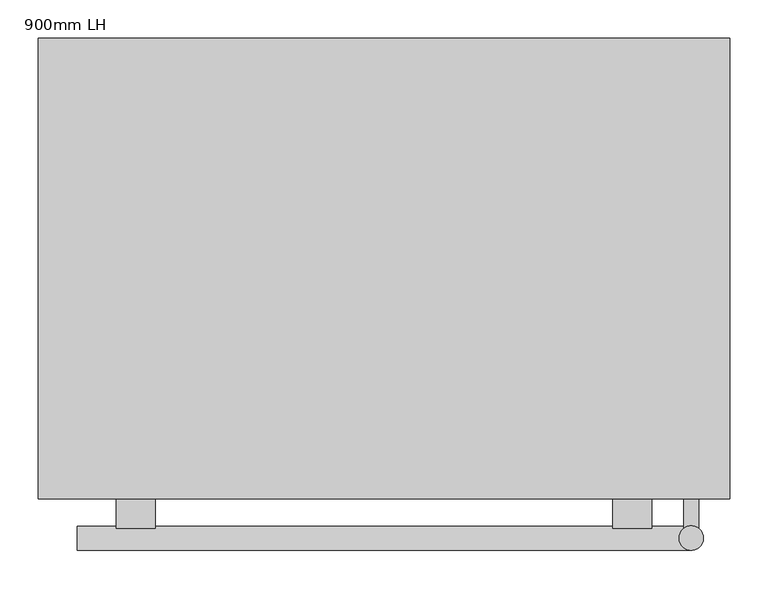
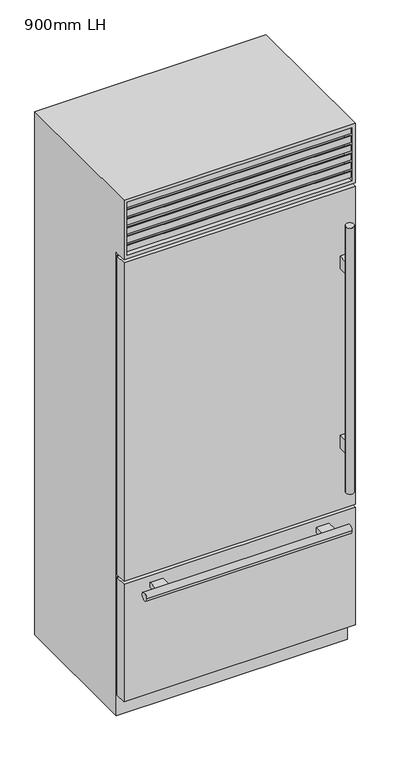
"""IFC4 building model written with IfcOpenShell, lengths in millimetres: proxy geometry, Refrigerador-combinado : 900mm LH."""

import ifcopenshell
import ifcopenshell.guid

model = None  # the IFC model being written
_history = None  # IfcOwnerHistory: only IFC2X3 demands one
_inside = {}  # id of a spatial element -> (the spatial element, [elements in it])
_under = {}  # id of a project, library or spatial element -> (it, [spatial elements below it])
_declared = {}  # id of a project -> (the project, [libraries it declares])
_typed = {}  # id of a type object -> (the type object, [elements of that type])
_made_of = {}  # id of a material, layer set ... -> (it, [elements and type objects made of it])


def new_model(schema):
    """Start an empty IFC model of exactly this schema.

    Asked for "IFC4X3", IfcOpenShell would pick the latest addendum, in which some entities
    have other attributes; the version numbers below select the first issue.
    IFC2X3 requires an IfcOwnerHistory on every rooted entity: one is made here for all.
    """
    global model, _history
    if schema == "IFC4X3":
        model = ifcopenshell.file(schema_version=(4, 3, 0, 0))
    else:
        model = ifcopenshell.file(schema=schema)
    _inside.clear()
    _under.clear()
    _declared.clear()
    _typed.clear()
    _made_of.clear()
    _history = None
    if model.schema == "IFC2X3":
        org = make("IfcOrganization", Name="unknown")
        user = make(
            "IfcPersonAndOrganization",
            ThePerson=make("IfcPerson", FamilyName="unknown"),
            TheOrganization=org,
        )
        app = make(
            "IfcApplication",
            ApplicationDeveloper=org,
            Version="unknown",
            ApplicationFullName="unknown",
            ApplicationIdentifier="unknown",
        )
        _history = make(
            "IfcOwnerHistory",
            OwningUser=user,
            OwningApplication=app,
            ChangeAction="ADDED",
            CreationDate=0,
        )
    return model


def make(cls, **values):
    """One entity of the class cls with the attributes given. An attribute that is None is left unset."""
    return model.create_entity(
        cls, **{name: value for name, value in values.items() if value is not None}
    )


def rooted(cls, **values):
    """An entity with a GlobalId (a new one), such as an element, a storey or a relation."""
    return make(cls, GlobalId=ifcopenshell.guid.new(), OwnerHistory=_history, **values)


def si_unit(unit_type, name, prefix=None):
    """IfcSIUnit, for example si_unit("LENGTHUNIT", "METRE", prefix="MILLI")."""
    return make("IfcSIUnit", UnitType=unit_type, Prefix=prefix, Name=name)


def assignment(units):
    """IfcUnitAssignment: the units of a project."""
    return None if units is None else make("IfcUnitAssignment", Units=units)


def point(xyz):
    """IfcCartesianPoint."""
    return None if xyz is None else make("IfcCartesianPoint", Coordinates=xyz)


def direction(xyz):
    """IfcDirection."""
    return None if xyz is None else make("IfcDirection", DirectionRatios=xyz)


def frame(location, z_axis=None, x_axis=None):
    """IfcAxis2Placement3D, a coordinate frame: its origin and axes. An axis left out is left unset."""
    return make(
        "IfcAxis2Placement3D",
        Location=point(location),
        Axis=direction(z_axis),
        RefDirection=direction(x_axis),
    )


def origin():
    """The frame at (0, 0, 0) with its axes left unset."""
    return frame((0.0, 0.0, 0.0))


def place(relative_to, where):
    """IfcLocalPlacement: puts the frame where relative to a parent placement (None: the world)."""
    return make(
        "IfcLocalPlacement", PlacementRelTo=relative_to, RelativePlacement=where
    )


def context(
    kind, dimensions, precision=None, world=None, true_north=None, identifier=None
):
    """IfcGeometricRepresentationContext, for example the 3D "Model" context."""
    return make(
        "IfcGeometricRepresentationContext",
        ContextIdentifier=identifier,
        ContextType=kind,
        CoordinateSpaceDimension=dimensions,
        Precision=precision,
        WorldCoordinateSystem=world,
        TrueNorth=true_north,
    )


def project(units=None, contexts=None):
    """IfcProject with its units and contexts."""
    return rooted(
        "IfcProject",
        Name="project",
        RepresentationContexts=contexts,
        UnitsInContext=assignment(units),
    )


def spatial(cls, under=None, at=None, **own):
    """A site, building, storey or space (cls), placed at a placement, below another one or the project."""
    s = rooted(cls, ObjectPlacement=at, **own)
    if under is not None:
        _under.setdefault(under.id(), (under, []))[1].append(s)
    return s


def polyline(points):
    """IfcPolyline through the points."""
    return make("IfcPolyline", Points=[point(p) for p in points])


def circle_curve(where, radius):
    """IfcCircle in the frame where."""
    return make("IfcCircle", Position=where, Radius=radius)


def ellipse_curve(where, semi_axis1, semi_axis2):
    """IfcEllipse in the frame where."""
    return make(
        "IfcEllipse", Position=where, SemiAxis1=semi_axis1, SemiAxis2=semi_axis2
    )


def outline(outer, holes=None, kind="AREA"):
    """IfcArbitraryClosedProfileDef: a profile drawn as a closed curve; with holes, ...WithVoids."""
    if holes is None:
        return make("IfcArbitraryClosedProfileDef", ProfileType=kind, OuterCurve=outer)
    return make(
        "IfcArbitraryProfileDefWithVoids",
        ProfileType=kind,
        OuterCurve=outer,
        InnerCurves=holes,
    )


def extrude(swept, where, along, depth):
    """IfcExtrudedAreaSolid: the profile swept, set in the frame where, extruded along a direction by depth."""
    return make(
        "IfcExtrudedAreaSolid",
        SweptArea=swept,
        Position=where,
        ExtrudedDirection=direction(along),
        Depth=depth,
    )


def faces_of(points, faces, orient=None, outer=None):
    """IfcFace entities. A face is a list of loops; a loop is a list of indices into points, from 0.

    orient and outer hold one flag for each loop. By default every Orientation is true, the
    first loop of a face is its IfcFaceOuterBound and the others are IfcFaceBound.
    """
    made = []
    for i, loops in enumerate(faces):
        bounds = []
        for j, loop in enumerate(loops):
            is_outer = j == 0 if outer is None else outer[i][j]
            bounds.append(
                make(
                    "IfcFaceOuterBound" if is_outer else "IfcFaceBound",
                    Bound=make("IfcPolyLoop", Polygon=[points[k] for k in loop]),
                    Orientation=True if orient is None else orient[i][j],
                )
            )
        made.append(make("IfcFace", Bounds=bounds))
    return made


def faceted_brep(points, faces, orient=None, outer=None, voids=None):
    """IfcFacetedBrep: a solid bounded by flat faces; with voids (closed shells), ...WithVoids."""
    shared = [point(p) for p in points]
    hull = make("IfcClosedShell", CfsFaces=faces_of(shared, faces, orient, outer))
    if voids is None:
        return make("IfcFacetedBrep", Outer=hull)
    return make(
        "IfcFacetedBrepWithVoids",
        Outer=hull,
        Voids=[
            make(cls, CfsFaces=faces_of(shared, fs, o, b)) for cls, fs, o, b in voids
        ],
    )


def shape(context_of_items, identifier, shape_type, items):
    """IfcShapeRepresentation: the items that make up one representation, for example the "Body"."""
    return make(
        "IfcShapeRepresentation",
        ContextOfItems=context_of_items,
        RepresentationIdentifier=identifier,
        RepresentationType=shape_type,
        Items=items,
    )


def source(mapping_origin, context_of_items, identifier, shape_type, items):
    """IfcRepresentationMap: a shape defined once, which mapped items show again and again."""
    return make(
        "IfcRepresentationMap",
        MappingOrigin=mapping_origin,
        MappedRepresentation=shape(context_of_items, identifier, shape_type, items),
    )


def transform(
    local_origin,
    x_axis=None,
    y_axis=None,
    z_axis=None,
    scale=None,
    scale2=None,
    scale3=None,
    uniform=True,
):
    """IfcCartesianTransformationOperator3D, or its non-uniform kind. x_axis, y_axis, z_axis: its Axis1, 2, 3."""
    if uniform:
        return make(
            "IfcCartesianTransformationOperator3D",
            Axis1=direction(x_axis),
            Axis2=direction(y_axis),
            LocalOrigin=point(local_origin),
            Scale=scale,
            Axis3=direction(z_axis),
        )
    return make(
        "IfcCartesianTransformationOperator3DnonUniform",
        Axis1=direction(x_axis),
        Axis2=direction(y_axis),
        LocalOrigin=point(local_origin),
        Scale=scale,
        Axis3=direction(z_axis),
        Scale2=scale2,
        Scale3=scale3,
    )


def mapped(mapping_source, mapping_target):
    """IfcMappedItem: shows the shape of a source again, moved by a transform."""
    return make(
        "IfcMappedItem", MappingSource=mapping_source, MappingTarget=mapping_target
    )


def made_of(thing, what):
    """Note that an element or type object is made of a material, layer set ...; save() writes the relation."""
    if what is not None:
        _made_of.setdefault(what.id(), (what, []))[1].append(thing)
    return thing


def element(
    cls,
    number,
    at=None,
    inside=None,
    cuts=None,
    type_object=None,
    material=None,
    context=None,
    identifier="Body",
    shape_type=None,
    held_by="IfcProductDefinitionShape",
    body=None,
    shapes=None,
    **own,
):
    """One element of the class cls, such as IfcWall. Its Tag is "e" and its number.

    at: its placement. inside: the storey or other place that contains it. cuts: it is an
    opening in that element (IfcRelVoidsElement). A single representation is given by context,
    identifier, shape_type and body (its items); several are given by shapes. held_by: the class
    of the entity that holds the representations. save() writes the other relations.
    """
    e = rooted(cls, Tag="e%d" % number, ObjectPlacement=at, **own)
    if body is not None:
        shapes = [shape(context, identifier, shape_type, body)]
    if shapes is not None:
        e.Representation = make(held_by, Representations=shapes)
    if inside is not None:
        _inside.setdefault(inside.id(), (inside, []))[1].append(e)
    if cuts is not None:
        rooted(
            "IfcRelVoidsElement", RelatingBuildingElement=cuts, RelatedOpeningElement=e
        )
    if type_object is not None:
        _typed.setdefault(type_object.id(), (type_object, []))[1].append(e)
    return made_of(e, material)


def aggregate(whole, parts):
    """IfcRelAggregates: a whole, such as a stair, and the parts it consists of."""
    return rooted("IfcRelAggregates", RelatingObject=whole, RelatedObjects=parts)


def save(model, path):
    """Write the relations noted so far, then the file.

    IfcRelAggregates (storeys below a building ...), IfcRelContainedInSpatialStructure (elements
    in a storey), IfcRelDefinesByType, IfcRelAssociatesMaterial and IfcRelDeclares: one each for
    every whole, place, type object, material and project.
    """
    for whole, parts in _under.values():
        aggregate(whole, parts)
    for where, things in _inside.values():
        rooted(
            "IfcRelContainedInSpatialStructure",
            RelatedElements=things,
            RelatingStructure=where,
        )
    for kind, things in _typed.values():
        rooted("IfcRelDefinesByType", RelatedObjects=things, RelatingType=kind)
    for what, things in _made_of.values():
        rooted("IfcRelAssociatesMaterial", RelatedObjects=things, RelatingMaterial=what)
    for by, libraries in _declared.values():
        rooted("IfcRelDeclares", RelatingContext=by, RelatedDefinitions=libraries)
    model.write(path)


def plane_surface(at):
    """IfcPlane: the flat surface through the origin of the frame at, square to its z axis."""
    return make("IfcPlane", Position=at)


def cylinder_surface(at, radius):
    """IfcCylindricalSurface: all points at the distance radius from the z axis of the frame at."""
    return make("IfcCylindricalSurface", Position=at, Radius=radius)


def advanced_brep(points, edges, surfaces, faces):
    """IfcAdvancedBrep: a solid bounded by faces that lie on surfaces and meet in shared edges.

    An edge is (start, end): straight between two places in points (the first is 0);
    or (start, end, curve); or (start, end, curve, False) where it runs against its curve.
    A face is (place in surfaces, loops), or (place, loops, False) where it looks against
    its surface's normal. A loop lists edges by number (the first is 1), with a minus sign
    where the edge is run from its end to its start. The first loop is the outer one.
    """
    corners = [point(p) for p in points]
    vertices = [make("IfcVertexPoint", VertexGeometry=c) for c in corners]
    made = []
    for start, end, *more in edges:
        made.append(
            make(
                "IfcEdgeCurve",
                EdgeStart=vertices[start],
                EdgeEnd=vertices[end],
                EdgeGeometry=more[0] if more else make("IfcPolyline", Points=[corners[start], corners[end]]),
                SameSense=more[1] if len(more) > 1 else True,
            )
        )
    hull = []
    for where, loops, *sense in faces:
        bounds = []
        for j, loop in enumerate(loops):
            ring = [make("IfcOrientedEdge", EdgeElement=made[abs(k) - 1], Orientation=k > 0) for k in loop]
            bounds.append(
                make(
                    "IfcFaceOuterBound" if j == 0 else "IfcFaceBound",
                    Bound=make("IfcEdgeLoop", EdgeList=ring),
                    Orientation=True,
                )
            )
        hull.append(make("IfcAdvancedFace", Bounds=bounds, FaceSurface=surfaces[where], SameSense=sense[0] if sense else True))
    return make("IfcAdvancedBrep", Outer=make("IfcClosedShell", CfsFaces=hull))


def proxy_900mm_lh_87200827(model_context):
    return source(origin(), model_context, "Body", "SolidModel", [
        extrude(outline(polyline([(-450.0, -655.55), (450.0, -655.55), (450.0, -700.0), (-450.0, -700.0), (-450.0, -655.55)])), frame((0.0, 0.0, 584.2), z_axis=(0.0, 0.0, 1.0), x_axis=(1.0, 0.0, 0.0)), (0.0, 0.0, 1.0), 1308.625),
        extrude(outline(polyline([(-450.0, -655.55), (450.0, -655.55), (450.0, -700.0), (-450.0, -700.0), (-450.0, -655.55)])), frame((0.0, 0.0, 88.9), z_axis=(0.0, 0.0, 1.0), x_axis=(1.0, 0.0, 0.0)), (0.0, 0.0, 1.0), 482.6),
        faceted_brep([(450.0, -700.0, 2150.0), (-450.0, -700.0, 2150.0), (-450.0, -700.0, 1905.525), (450.0, -700.0, 1905.525), (437.3, -700.0, 2137.3), (437.3, -700.0, 1918.225), (-437.3, -700.0, 1918.225), (-437.3, -700.0, 2137.3), (450.0, -100.0, 2150.0), (-450.0, -100.0, 2150.0), (-450.0, -100.0, 0.0), (-450.0, -649.2, 0.0), (-450.0, -649.2, 1905.525), (450.0, -649.2, 1905.525), (450.0, -649.2, 0.0), (450.0, -100.0, 0.0), (-437.3, -649.2, 2137.3), (437.3, -649.2, 2137.3), (-437.3, -649.2, 1918.225), (437.3, -649.2, 1918.225)], [[[0, 1, 2, 3], [4, 5, 6, 7]], [[1, 0, 8, 9]], [[2, 1, 9, 10, 11, 12]], [[3, 2, 12, 13]], [[8, 0, 3, 13, 14, 15]], [[4, 7, 16, 17]], [[7, 6, 18, 16]], [[6, 5, 19, 18]], [[5, 4, 17, 19]], [[15, 14, 11, 10]], [[9, 8, 15, 10]], [[17, 16, 18, 19]], [[11, 14, 13, 12]]]),
        extrude(outline(polyline([(-649.2, 1918.225), (-696.825, 1930.9860803), (-696.825, 1956.3860803), (-693.65, 1956.3860803), (-693.65, 1933.5368938), (-649.2, 1921.6265522), (-649.2, 1918.225)])), frame((-437.3, 0.0, 0.0), z_axis=(1.0, 0.0, 0.0), x_axis=(0.0, 1.0, 0.0)), (0.0, 0.0, 1.0), 874.6),
        extrude(outline(polyline([(-649.2, 1954.4077839), (-696.825, 1967.1688642), (-696.825, 1992.5688642), (-693.65, 1992.5688642), (-693.65, 1969.7196777), (-649.2, 1957.8093361), (-649.2, 1954.4077839)])), frame((-437.3, 0.0, 0.0), z_axis=(1.0, 0.0, 0.0), x_axis=(0.0, 1.0, 0.0)), (0.0, 0.0, 1.0), 874.6),
        extrude(outline(polyline([(-649.2, 1990.5905679), (-696.825, 2003.3516482), (-696.825, 2028.7516482), (-693.65, 2028.7516482), (-693.65, 2005.9024616), (-649.2, 1993.99212), (-649.2, 1990.5905679)])), frame((-437.3, 0.0, 0.0), z_axis=(1.0, 0.0, 0.0), x_axis=(0.0, 1.0, 0.0)), (0.0, 0.0, 1.0), 874.6),
        extrude(outline(polyline([(-649.2, 2026.7733518), (-696.825, 2039.5344321), (-696.825, 2064.9344321), (-693.65, 2064.9344321), (-693.65, 2042.0852456), (-649.2, 2030.174904), (-649.2, 2026.7733518)])), frame((-437.3, 0.0, 0.0), z_axis=(1.0, 0.0, 0.0), x_axis=(0.0, 1.0, 0.0)), (0.0, 0.0, 1.0), 874.6),
        extrude(outline(polyline([(-649.2, 2062.9561358), (-696.825, 2075.7172161), (-696.825, 2101.1172161), (-693.65, 2101.1172161), (-693.65, 2078.2680295), (-649.2, 2066.3576879), (-649.2, 2062.9561358)])), frame((-437.3, 0.0, 0.0), z_axis=(1.0, 0.0, 0.0), x_axis=(0.0, 1.0, 0.0)), (0.0, 0.0, 1.0), 874.6),
        extrude(outline(polyline([(-649.2, 2099.1389197), (-696.825, 2111.9), (-696.825, 2137.3), (-693.65, 2137.3), (-693.65, 2114.4508135), (-649.2, 2102.5404719), (-649.2, 2099.1389197)])), frame((-437.3, 0.0, 0.0), z_axis=(1.0, 0.0, 0.0), x_axis=(0.0, 1.0, 0.0)), (0.0, 0.0, 1.0), 874.6),
        advanced_brep(
        [(-443.65, -649.2, 565.15), (-443.65, -655.55, 565.15), (-443.65, -655.55, 95.25), (-443.65, -649.2, 95.25), (-446.825, -655.55, 568.325), (-446.825, -649.2, 568.325), (-446.825, -649.2, 92.075), (-446.825, -655.55, 92.075), (443.65, -655.55, 95.25), (443.65, -649.2, 95.25), (446.825, -649.2, 92.075), (446.825, -655.55, 92.075), (443.65, -655.55, 565.15), (443.65, -649.2, 565.15), (446.825, -649.2, 568.325), (446.825, -655.55, 568.325)],
        [
            (0, 1),
            (1, 2),
            (2, 3),
            (3, 0),
            (4, 5, ellipse_curve(frame((-446.825, -652.375, 568.325), z_axis=(-0.7071067811865475, 0.0, -0.7071067811865476), x_axis=(-0.7071067811865476, 0.0, 0.7071067811865475)), 4.4901281, 3.175)),
            (5, 6),
            (6, 7, ellipse_curve(frame((-446.825, -652.375, 92.075), z_axis=(-0.7071067811865475, 0.0, 0.7071067811865475), x_axis=(0.7071067811865474, 0.0, 0.7071067811865477)), 4.4901281, 3.175)),
            (7, 4),
            (2, 8),
            (8, 9),
            (9, 3),
            (6, 10),
            (10, 11, ellipse_curve(frame((446.825, -652.375, 92.075), z_axis=(-0.7071067811865475, 0.0, -0.7071067811865476), x_axis=(-0.7071067811865476, 0.0, 0.7071067811865474)), 4.4901281, 3.175)),
            (11, 7),
            (8, 12),
            (12, 13),
            (13, 9),
            (10, 14),
            (14, 15, ellipse_curve(frame((446.825, -652.375, 568.325), z_axis=(0.7071067811865476, 0.0, -0.7071067811865474), x_axis=(-0.7071067811865474, 0.0, -0.7071067811865477)), 4.4901281, 3.175)),
            (15, 11),
            (12, 1),
            (0, 13),
            (5, 14),
            (4, 15),
        ],
        [
            plane_surface(frame((-443.65, -655.55, 565.15), z_axis=(1.0, 0.0, 0.0), x_axis=(0.0, 0.0, -1.0))),
            cylinder_surface(frame((-446.825, -652.375, 571.5), z_axis=(0.0, 0.0, 1.0), x_axis=(0.0, -1.0, 0.0)), 3.175),
            plane_surface(frame((-443.65, -655.55, 95.25), z_axis=(0.0, 0.0, 1.0), x_axis=(1.0, 0.0, 0.0))),
            cylinder_surface(frame((-450.0, -652.375, 92.075), z_axis=(-1.0, 0.0, 0.0), x_axis=(0.0, -1.0, 0.0)), 3.175),
            plane_surface(frame((443.65, -655.55, 95.25), z_axis=(-1.0, 0.0, 0.0), x_axis=(0.0, 0.0, 1.0))),
            cylinder_surface(frame((446.825, -652.375, 88.9), z_axis=(0.0, 0.0, -1.0), x_axis=(0.0, -1.0, 0.0)), 3.175),
            plane_surface(frame((443.65, -655.55, 565.15), z_axis=(0.0, 0.0, -1.0), x_axis=(-1.0, 0.0, 0.0))),
            plane_surface(frame((443.65, -649.2, 565.15), z_axis=(0.0, 1.0, 0.0), x_axis=(-1.0, 0.0, 0.0))),
            cylinder_surface(frame((450.0, -652.375, 568.325), z_axis=(1.0, 0.0, 0.0), x_axis=(0.0, -1.0, 0.0)), 3.175),
            plane_surface(frame((446.825, -655.55, 568.325), z_axis=(0.0, -1.0, 0.0), x_axis=(-1.0, 0.0, 0.0))),
        ],
        [
            (0, [[1, 2, 3, 4]]),
            (1, [[5, 6, 7, 8]]),
            (2, [[-3, 9, 10, 11]]),
            (3, [[-7, 12, 13, 14]]),
            (4, [[-10, 15, 16, 17]]),
            (5, [[-13, 18, 19, 20]]),
            (6, [[-16, 21, -1, 22]]),
            (7, [[23, -18, -12, -6], [-11, -17, -22, -4]]),
            (8, [[-19, -23, -5, 24]]),
            (9, [[-14, -20, -24, -8], [-21, -15, -9, -2]]),
        ],
    ),
        advanced_brep(
        [(-443.65, -649.2, 1886.475), (-443.65, -655.55, 1886.475), (-443.65, -655.55, 590.55), (-443.65, -649.2, 590.55), (-446.825, -655.55, 1889.65), (-446.825, -649.2, 1889.65), (-446.825, -649.2, 587.375), (-446.825, -655.55, 587.375), (443.65, -655.55, 590.55), (443.65, -649.2, 590.55), (446.825, -649.2, 587.375), (446.825, -655.55, 587.375), (443.65, -655.55, 1886.475), (443.65, -649.2, 1886.475), (446.825, -649.2, 1889.65), (446.825, -655.55, 1889.65)],
        [
            (0, 1),
            (1, 2),
            (2, 3),
            (3, 0),
            (4, 5, ellipse_curve(frame((-446.825, -652.375, 1889.65), z_axis=(-0.7071067811865476, 0.0, -0.7071067811865475), x_axis=(-0.7071067811865475, 0.0, 0.7071067811865475)), 4.4901281, 3.175)),
            (5, 6),
            (6, 7, ellipse_curve(frame((-446.825, -652.375, 587.375), z_axis=(-0.7071067811865475, 0.0, 0.7071067811865476), x_axis=(0.7071067811865475, 0.0, 0.7071067811865475)), 4.4901281, 3.175)),
            (7, 4),
            (2, 8),
            (8, 9),
            (9, 3),
            (6, 10),
            (10, 11, ellipse_curve(frame((446.825, -652.375, 587.375), z_axis=(-0.7071067811865476, 0.0, -0.7071067811865475), x_axis=(-0.7071067811865475, 0.0, 0.7071067811865475)), 4.4901281, 3.175)),
            (11, 7),
            (8, 12),
            (12, 13),
            (13, 9),
            (10, 14),
            (14, 15, ellipse_curve(frame((446.825, -652.375, 1889.65), z_axis=(0.7071067811865474, 0.0, -0.7071067811865476), x_axis=(-0.7071067811865475, 0.0, -0.7071067811865476)), 4.4901281, 3.175)),
            (15, 11),
            (12, 1),
            (0, 13),
            (5, 14),
            (4, 15),
        ],
        [
            plane_surface(frame((-443.65, -655.55, 1886.475), z_axis=(1.0, 0.0, 0.0), x_axis=(0.0, 0.0, -1.0))),
            cylinder_surface(frame((-446.825, -652.375, 1892.825), z_axis=(0.0, 0.0, 1.0), x_axis=(0.0, -1.0, 0.0)), 3.175),
            plane_surface(frame((-443.65, -655.55, 590.55), z_axis=(0.0, 0.0, 1.0), x_axis=(1.0, 0.0, 0.0))),
            cylinder_surface(frame((-450.0, -652.375, 587.375), z_axis=(-1.0, 0.0, 0.0), x_axis=(0.0, -1.0, 0.0)), 3.175),
            plane_surface(frame((443.65, -655.55, 590.55), z_axis=(-1.0, 0.0, 0.0), x_axis=(0.0, 0.0, 1.0))),
            cylinder_surface(frame((446.825, -652.375, 584.2), z_axis=(0.0, 0.0, -1.0), x_axis=(0.0, -1.0, 0.0)), 3.175),
            plane_surface(frame((443.65, -655.55, 1886.475), z_axis=(0.0, 0.0, -1.0), x_axis=(-1.0, 0.0, 0.0))),
            plane_surface(frame((443.65, -649.2, 1886.475), z_axis=(0.0, 1.0, 0.0), x_axis=(-1.0, 0.0, 0.0))),
            cylinder_surface(frame((450.0, -652.375, 1889.65), z_axis=(1.0, 0.0, 0.0), x_axis=(0.0, -1.0, 0.0)), 3.175),
            plane_surface(frame((446.825, -655.55, 1889.65), z_axis=(0.0, -1.0, 0.0), x_axis=(-1.0, 0.0, 0.0))),
        ],
        [
            (0, [[1, 2, 3, 4]]),
            (1, [[5, 6, 7, 8]]),
            (2, [[-3, 9, 10, 11]]),
            (3, [[-7, 12, 13, 14]]),
            (4, [[-10, 15, 16, 17]]),
            (5, [[-13, 18, 19, 20]]),
            (6, [[-16, 21, -1, 22]]),
            (7, [[23, -18, -12, -6], [-11, -17, -22, -4]]),
            (8, [[-19, -23, -5, 24]]),
            (9, [[-14, -20, -24, -8], [-21, -15, -9, -2]]),
        ],
    ),
        advanced_brep(
        [(-297.6, -700.0, 542.925), (-297.6, -700.0, 523.875), (-348.4, -700.0, 523.875), (-348.4, -700.0, 542.925), (297.6, -700.0, 542.925), (348.4, -700.0, 542.925), (348.4, -700.0, 523.875), (297.6, -700.0, 523.875), (-297.6, -738.4741958, 542.925), (-297.6, -735.2991958, 533.4), (-297.6, -738.4741958, 523.875), (-348.4, -738.4741958, 523.875), (-348.4, -735.2991958, 533.4), (-348.4, -738.4741958, 542.925), (297.6, -738.4741958, 542.925), (348.4, -738.4741958, 542.925), (348.4, -735.2991958, 533.4), (348.4, -738.4741958, 523.875), (297.6, -738.4741958, 523.875), (297.6, -735.2991958, 533.4), (399.2, -767.0491958, 533.4), (399.2, -735.2991958, 533.4), (-399.2, -767.0491958, 533.4), (-399.2, -735.2991958, 533.4)],
        [
            (0, 1),
            (1, 2),
            (2, 3),
            (3, 0),
            (4, 5),
            (5, 6),
            (6, 7),
            (7, 4),
            (0, 8),
            (8, 9, circle_curve(frame((-297.6, -751.1741958, 533.4), z_axis=(-1.0, 0.0, 0.0), x_axis=(0.0, 1.0, 0.0)), 15.875)),
            (9, 10, circle_curve(frame((-297.6, -751.1741958, 533.4), z_axis=(-1.0, 0.0, 0.0), x_axis=(0.0, 1.0, 0.0)), 15.875)),
            (10, 1),
            (10, 11),
            (11, 2),
            (11, 12, circle_curve(frame((-348.4, -751.1741958, 533.4), z_axis=(1.0, 0.0, 0.0), x_axis=(0.0, 1.0, 0.0)), 15.875)),
            (12, 13, circle_curve(frame((-348.4, -751.1741958, 533.4), z_axis=(1.0, 0.0, 0.0), x_axis=(0.0, 1.0, 0.0)), 15.875)),
            (13, 3),
            (13, 8),
            (4, 14),
            (14, 15),
            (15, 5),
            (15, 16, circle_curve(frame((348.4, -751.1741958, 533.4), z_axis=(-1.0, 0.0, 0.0), x_axis=(0.0, 1.0, 0.0)), 15.875)),
            (16, 17, circle_curve(frame((348.4, -751.1741958, 533.4), z_axis=(-1.0, 0.0, 0.0), x_axis=(0.0, 1.0, 0.0)), 15.875)),
            (17, 6),
            (17, 18),
            (18, 7),
            (18, 19, circle_curve(frame((297.6, -751.1741958, 533.4), z_axis=(1.0, 0.0, 0.0), x_axis=(0.0, 1.0, 0.0)), 15.875)),
            (19, 14, circle_curve(frame((297.6, -751.1741958, 533.4), z_axis=(1.0, 0.0, 0.0), x_axis=(0.0, 1.0, 0.0)), 15.875)),
            (20, 21, circle_curve(frame((399.2, -751.1741958, 533.4), z_axis=(1.0, 0.0, 0.0), x_axis=(0.0, 1.0, 0.0)), 15.875)),
            (21, 20, circle_curve(frame((399.2, -751.1741958, 533.4), z_axis=(1.0, 0.0, 0.0), x_axis=(0.0, 1.0, 0.0)), 15.875)),
            (22, 23, circle_curve(frame((-399.2, -751.1741958, 533.4), z_axis=(-1.0, 0.0, 0.0), x_axis=(0.0, 1.0, 0.0)), 15.875)),
            (23, 22, circle_curve(frame((-399.2, -751.1741958, 533.4), z_axis=(-1.0, 0.0, 0.0), x_axis=(0.0, 1.0, 0.0)), 15.875)),
            (20, 22),
            (23, 12),
            (9, 19),
            (16, 21),
        ],
        [
            plane_surface(frame((-297.6, -700.0, 542.925), z_axis=(0.0, 1.0, 0.0), x_axis=(0.0, 0.0, -1.0))),
            plane_surface(frame((-297.6, -700.0, 542.925), z_axis=(1.0, 0.0, 0.0), x_axis=(0.0, -1.0, 0.0))),
            plane_surface(frame((-297.6, -700.0, 523.875), z_axis=(0.0, 0.0, -1.0), x_axis=(0.0, -1.0, 0.0))),
            plane_surface(frame((-348.4, -700.0, 523.875), z_axis=(-1.0, 0.0, 0.0), x_axis=(0.0, -1.0, 0.0))),
            plane_surface(frame((-348.4, -700.0, 542.925), z_axis=(0.0, 0.0, 1.0), x_axis=(0.0, -1.0, 0.0))),
            plane_surface(frame((297.6, -700.0, 542.925), z_axis=(0.0, 0.0, 1.0), x_axis=(0.0, -1.0, 0.0))),
            plane_surface(frame((348.4, -700.0, 542.925), z_axis=(1.0, 0.0, 0.0), x_axis=(0.0, -1.0, 0.0))),
            plane_surface(frame((348.4, -700.0, 523.875), z_axis=(0.0, 0.0, -1.0), x_axis=(0.0, -1.0, 0.0))),
            plane_surface(frame((297.6, -700.0, 523.875), z_axis=(-1.0, 0.0, 0.0), x_axis=(0.0, -1.0, 0.0))),
            plane_surface(frame((399.2, -735.2991958, 533.4), z_axis=(1.0, 0.0, 0.0), x_axis=(0.0, 0.0, 1.0))),
            plane_surface(frame((-399.2, -735.2991958, 533.4), z_axis=(-1.0, 0.0, 0.0), x_axis=(0.0, 0.0, -1.0))),
            cylinder_surface(frame((-399.2, -751.1741958, 533.4), z_axis=(1.0, 0.0, 0.0), x_axis=(0.0, 1.0, 0.0)), 15.875),
        ],
        [
            (0, [[1, 2, 3, 4]]),
            (0, [[5, 6, 7, 8]]),
            (1, [[-1, 9, 10, 11, 12]]),
            (2, [[-2, -12, 13, 14]]),
            (3, [[-3, -14, 15, 16, 17]]),
            (4, [[-4, -17, 18, -9]]),
            (5, [[-5, 19, 20, 21]]),
            (6, [[-6, -21, 22, 23, 24]]),
            (7, [[-7, -24, 25, 26]]),
            (8, [[-8, -26, 27, 28, -19]]),
            (9, [[29, 30]]),
            (10, [[31, 32]]),
            (11, [[-29, 33, -32, 34, -15, -13, -11, 35, -27, -25, -23, 36]]),
            (11, [[-30, -36, -22, -20, -28, -35, -10, -18, -16, -34, -31, -33]]),
        ],
    ),
        advanced_brep(
        [(409.525, -700.0, 1626.125), (409.525, -700.0, 1575.325), (390.475, -700.0, 1575.325), (390.475, -700.0, 1626.125), (409.525, -700.0, 889.0), (409.525, -700.0, 838.2), (390.475, -700.0, 838.2), (390.475, -700.0, 889.0), (409.525, -738.4741958, 1626.125), (409.525, -738.4741958, 1575.325), (390.475, -738.4741958, 1575.325), (390.475, -738.4741958, 1626.125), (409.525, -738.4741958, 889.0), (409.525, -738.4741958, 838.2), (390.475, -738.4741958, 838.2), (390.475, -738.4741958, 889.0), (384.125, -751.1741958, 1778.525), (415.875, -751.1741958, 1778.525), (384.125, -751.1741958, 685.8), (415.875, -751.1741958, 685.8)],
        [
            (0, 1),
            (1, 2),
            (2, 3),
            (3, 0),
            (4, 5),
            (5, 6),
            (6, 7),
            (7, 4),
            (0, 8),
            (8, 9),
            (9, 1),
            (9, 10, circle_curve(frame((400.0, -751.1741958, 1575.325), z_axis=(0.0, 0.0, 1.0), x_axis=(1.0, 0.0, 0.0)), 15.875)),
            (10, 2),
            (10, 11),
            (11, 3),
            (11, 8, circle_curve(frame((400.0, -751.1741958, 1626.125), z_axis=(0.0, 0.0, -1.0), x_axis=(1.0, 0.0, 0.0)), 15.875)),
            (4, 12),
            (12, 13),
            (13, 5),
            (13, 14, circle_curve(frame((400.0, -751.1741958, 838.2), z_axis=(0.0, 0.0, 1.0), x_axis=(1.0, 0.0, 0.0)), 15.875)),
            (14, 6),
            (14, 15),
            (15, 7),
            (15, 12, circle_curve(frame((400.0, -751.1741958, 889.0), z_axis=(0.0, 0.0, -1.0), x_axis=(1.0, 0.0, 0.0)), 15.875)),
            (16, 17, circle_curve(frame((400.0, -751.1741958, 1778.525), z_axis=(0.0, 0.0, 1.0), x_axis=(1.0, 0.0, 0.0)), 15.875)),
            (17, 16, circle_curve(frame((400.0, -751.1741958, 1778.525), z_axis=(0.0, 0.0, 1.0), x_axis=(1.0, 0.0, 0.0)), 15.875)),
            (18, 19, circle_curve(frame((400.0, -751.1741958, 685.8), z_axis=(0.0, 0.0, -1.0), x_axis=(1.0, 0.0, 0.0)), 15.875)),
            (19, 18, circle_curve(frame((400.0, -751.1741958, 685.8), z_axis=(0.0, 0.0, -1.0), x_axis=(1.0, 0.0, 0.0)), 15.875)),
            (16, 18),
            (19, 17),
        ],
        [
            plane_surface(frame((409.525, -700.0, 1626.125), z_axis=(0.0, 1.0, 0.0), x_axis=(0.0, 0.0, -1.0))),
            plane_surface(frame((409.525, -700.0, 1626.125), z_axis=(1.0, 0.0, 0.0), x_axis=(0.0, -1.0, 0.0))),
            plane_surface(frame((409.525, -700.0, 1575.325), z_axis=(0.0, 0.0, -1.0), x_axis=(0.0, -1.0, 0.0))),
            plane_surface(frame((390.475, -700.0, 1575.325), z_axis=(-1.0, 0.0, 0.0), x_axis=(0.0, -1.0, 0.0))),
            plane_surface(frame((390.475, -700.0, 1626.125), z_axis=(0.0, 0.0, 1.0), x_axis=(0.0, -1.0, 0.0))),
            plane_surface(frame((409.525, -700.0, 889.0), z_axis=(1.0, 0.0, 0.0), x_axis=(0.0, -1.0, 0.0))),
            plane_surface(frame((409.525, -700.0, 838.2), z_axis=(0.0, 0.0, -1.0), x_axis=(0.0, -1.0, 0.0))),
            plane_surface(frame((390.475, -700.0, 838.2), z_axis=(-1.0, 0.0, 0.0), x_axis=(0.0, -1.0, 0.0))),
            plane_surface(frame((390.475, -700.0, 889.0), z_axis=(0.0, 0.0, 1.0), x_axis=(0.0, -1.0, 0.0))),
            plane_surface(frame((415.875, -751.1741958, 1778.525), z_axis=(0.0, 0.0, 1.0), x_axis=(0.0, 1.0, 0.0))),
            plane_surface(frame((415.875, -751.1741958, 685.8), z_axis=(0.0, 0.0, -1.0), x_axis=(0.0, -1.0, 0.0))),
            cylinder_surface(frame((400.0, -751.1741958, 685.8), z_axis=(0.0, 0.0, 1.0), x_axis=(1.0, 0.0, 0.0)), 15.875),
        ],
        [
            (0, [[1, 2, 3, 4]]),
            (0, [[5, 6, 7, 8]]),
            (1, [[-1, 9, 10, 11]]),
            (2, [[-2, -11, 12, 13]]),
            (3, [[-3, -13, 14, 15]]),
            (4, [[-4, -15, 16, -9]]),
            (5, [[-5, 17, 18, 19]]),
            (6, [[-6, -19, 20, 21]]),
            (7, [[-7, -21, 22, 23]]),
            (8, [[-8, -23, 24, -17]]),
            (9, [[25, 26]]),
            (10, [[27, 28]]),
            (11, [[-25, 29, -28, 30]]),
            (11, [[-26, -30, -27, -29], [-10, -16, -14, -12], [-18, -24, -22, -20]]),
        ],
    ),
    ])


if __name__ == "__main__":
    model = new_model("IFC4")
    model_context = context("Model", 3, world=origin())
    ifc_project = project(units=[si_unit("LENGTHUNIT", "METRE", prefix="MILLI")], contexts=[model_context])
    site = spatial("IfcSite", under=ifc_project)
    building = spatial("IfcBuilding", under=site)
    placement = place(None, origin())
    proxy_900mm_lh_shape = proxy_900mm_lh_87200827(model_context)
    element("IfcBuildingElementProxy", 1, Name="Refrigerador-combinado : 900mm LH", ObjectType="Refrigerador-combinado : 900mm LH", at=placement, inside=building, context=model_context, shape_type="MappedRepresentation", body=[
        mapped(proxy_900mm_lh_shape, transform((0.0, 0.0, 0.0), x_axis=(1.0, 0.0, 0.0), y_axis=(0.0, 1.0, 0.0), z_axis=(0.0, 0.0, 1.0))),
    ])
    save(model, "model.ifc")

# Revit data of these elements
# Project information
#   Data de emissão do projeto = "Data de emissão"
#   Status do projeto = "Status do projeto"
#   Nome do cliente = "Proprietário"
#   Endereço do projeto = "Insira aqui o endereço"
#   Nome do projeto = "Nome do projeto"
#   Número do projeto = "0001"
# Type "Refrigerador-combinado : 900mm LH"
#   Legenda = "Refrigerador"
#   Description = "Refrigerador combinado"
#   Assembly Code = "E1090320"
#   Largura = 900 mm
#   Deslocamento de parede = 100 mm
#   Voltagem = 120 V
#   Consumo de energia = 1000 VA
#   Altura = 2150 mm
#   Linha de centro do puxador = 850 mm
#   Linear = 600 mm
#   Amperagem = 8.33333 A
#   Mostrar legenda = yes
#   RH = no
#   LH = yes
#   Junta = Eletrodoméstico – Junta
#   Acabamento do eletrodoméstico = Eletrodoméstico – Aço inoxidável
#   Default Elevation = 0
# Element 1 (IfcBuildingElementProxy, "Refrigerador-combinado : 900mm LH")
#   Materials on its faces: "Eletrodoméstico – Aço inoxidável", "Eletrodoméstico – Junta"
# Materials
#   "Eletrodoméstico – Junta": class "Diversos", colour RGB 234 234 234, transparency 0, Cost = 0
#   "Eletrodoméstico – Aço inoxidável": class "Metal", colour RGB 189 187 185, transparency 0, Description = "Aço inoxidável 18/8", Cost = 0
